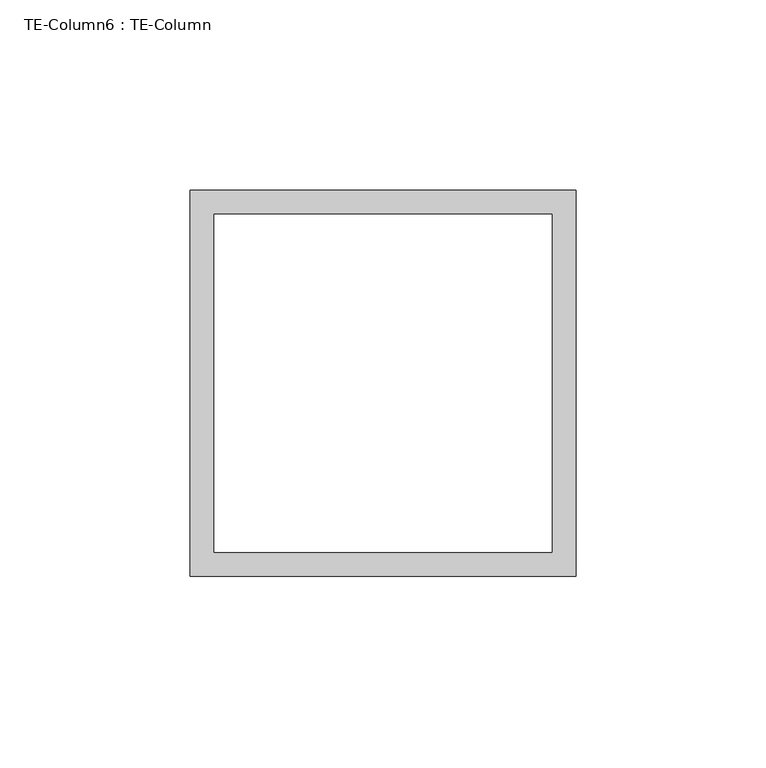
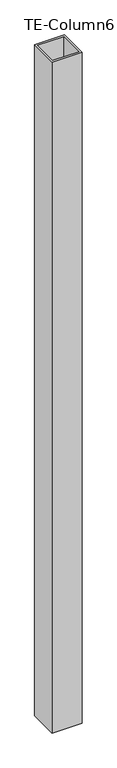
"""IFC4 building model written with IfcOpenShell, lengths in millimetres: proxy geometry, TE-Column6 : TE-Column."""

from ifc_helpers import new_model, si_unit, frame, origin, place, context, project, spatial, polyline, outline, extrude, source, transform, mapped, element, save


def te_column6_te_column_06b2476f(model_context):
    return source(origin(), model_context, "Body", "SweptSolid", [
        extrude(outline(polyline([(590318.6434739, -535255.5413841), (590217.0434739, -535255.5413841), (590217.0434739, -535153.9413841), (590318.6434739, -535153.9413841), (590318.6434739, -535255.5413841)]), holes=[polyline([(590312.2934739, -535160.2913841), (590223.3934739, -535160.2913841), (590223.3934739, -535249.1913841), (590312.2934739, -535249.1913841), (590312.2934739, -535160.2913841)])]), frame((0.0, 0.0, 28.575), z_axis=(0.0, 0.0, 1.0), x_axis=(1.0, 0.0, 0.0)), (0.0, 0.0, 1.0), 2406.65),
    ])


if __name__ == "__main__":
    model = new_model("IFC4")
    model_context = context("Model", 3, world=origin())
    ifc_project = project(units=[si_unit("LENGTHUNIT", "METRE", prefix="MILLI")], contexts=[model_context])
    site = spatial("IfcSite", under=ifc_project)
    building = spatial("IfcBuilding", under=site)
    placement = place(None, origin())
    te_column6_te_column_shape = te_column6_te_column_06b2476f(model_context)
    element("IfcBuildingElementProxy", 1, Name="TE-Column6 : TE-Column", ObjectType="TE-Column6 : TE-Column", at=placement, inside=building, context=model_context, shape_type="MappedRepresentation", body=[
        mapped(te_column6_te_column_shape, transform((0.0, 0.0, 0.0), x_axis=(1.0, 0.0, 0.0), y_axis=(0.0, 1.0, 0.0), z_axis=(0.0, 0.0, 1.0))),
    ])
    save(model, "model.ifc")

# Revit data of these elements
# Element 1 (IfcBuildingElementProxy, "TE-Column6 : TE-Column")
#   Materials on its faces: "4\"X4\" GALV. HSS TUBING"
# Materials
#   "4\"X4\" GALV. HSS TUBING": class "Generic", colour RGB 211 211 207, transparency 0, Cost = 0
